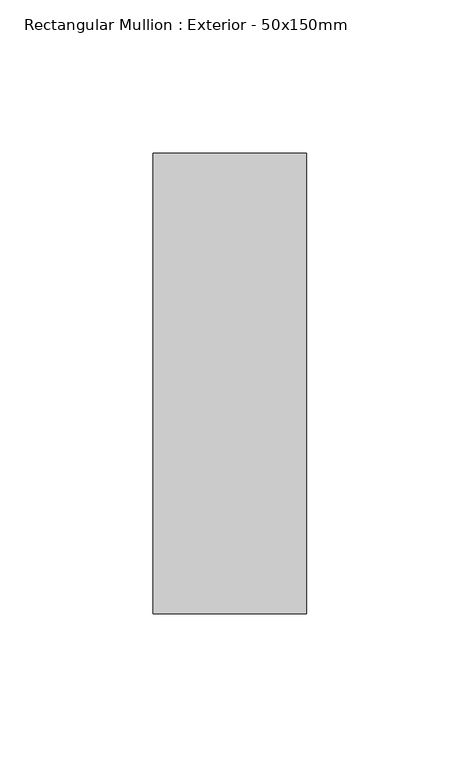
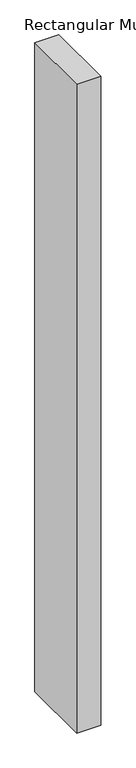
"""IFC4 building model written with IfcOpenShell, lengths in millimetres: member geometry, Rectangular Mullion : Exterior - 50x150mm."""

import ifcopenshell
import ifcopenshell.guid

model = None  # the IFC model being written
_history = None  # IfcOwnerHistory: only IFC2X3 demands one
_inside = {}  # id of a spatial element -> (the spatial element, [elements in it])
_under = {}  # id of a project, library or spatial element -> (it, [spatial elements below it])
_declared = {}  # id of a project -> (the project, [libraries it declares])
_typed = {}  # id of a type object -> (the type object, [elements of that type])
_made_of = {}  # id of a material, layer set ... -> (it, [elements and type objects made of it])


def new_model(schema):
    """Start an empty IFC model of exactly this schema.

    Asked for "IFC4X3", IfcOpenShell would pick the latest addendum, in which some entities
    have other attributes; the version numbers below select the first issue.
    IFC2X3 requires an IfcOwnerHistory on every rooted entity: one is made here for all.
    """
    global model, _history
    if schema == "IFC4X3":
        model = ifcopenshell.file(schema_version=(4, 3, 0, 0))
    else:
        model = ifcopenshell.file(schema=schema)
    _inside.clear()
    _under.clear()
    _declared.clear()
    _typed.clear()
    _made_of.clear()
    _history = None
    if model.schema == "IFC2X3":
        org = make("IfcOrganization", Name="unknown")
        user = make(
            "IfcPersonAndOrganization",
            ThePerson=make("IfcPerson", FamilyName="unknown"),
            TheOrganization=org,
        )
        app = make(
            "IfcApplication",
            ApplicationDeveloper=org,
            Version="unknown",
            ApplicationFullName="unknown",
            ApplicationIdentifier="unknown",
        )
        _history = make(
            "IfcOwnerHistory",
            OwningUser=user,
            OwningApplication=app,
            ChangeAction="ADDED",
            CreationDate=0,
        )
    return model


def make(cls, **values):
    """One entity of the class cls with the attributes given. An attribute that is None is left unset."""
    return model.create_entity(
        cls, **{name: value for name, value in values.items() if value is not None}
    )


def rooted(cls, **values):
    """An entity with a GlobalId (a new one), such as an element, a storey or a relation."""
    return make(cls, GlobalId=ifcopenshell.guid.new(), OwnerHistory=_history, **values)


def si_unit(unit_type, name, prefix=None):
    """IfcSIUnit, for example si_unit("LENGTHUNIT", "METRE", prefix="MILLI")."""
    return make("IfcSIUnit", UnitType=unit_type, Prefix=prefix, Name=name)


def assignment(units):
    """IfcUnitAssignment: the units of a project."""
    return None if units is None else make("IfcUnitAssignment", Units=units)


def point(xyz):
    """IfcCartesianPoint."""
    return None if xyz is None else make("IfcCartesianPoint", Coordinates=xyz)


def direction(xyz):
    """IfcDirection."""
    return None if xyz is None else make("IfcDirection", DirectionRatios=xyz)


def frame(location, z_axis=None, x_axis=None):
    """IfcAxis2Placement3D, a coordinate frame: its origin and axes. An axis left out is left unset."""
    return make(
        "IfcAxis2Placement3D",
        Location=point(location),
        Axis=direction(z_axis),
        RefDirection=direction(x_axis),
    )


def origin():
    """The frame at (0, 0, 0) with its axes left unset."""
    return frame((0.0, 0.0, 0.0))


def place(relative_to, where):
    """IfcLocalPlacement: puts the frame where relative to a parent placement (None: the world)."""
    return make(
        "IfcLocalPlacement", PlacementRelTo=relative_to, RelativePlacement=where
    )


def context(
    kind, dimensions, precision=None, world=None, true_north=None, identifier=None
):
    """IfcGeometricRepresentationContext, for example the 3D "Model" context."""
    return make(
        "IfcGeometricRepresentationContext",
        ContextIdentifier=identifier,
        ContextType=kind,
        CoordinateSpaceDimension=dimensions,
        Precision=precision,
        WorldCoordinateSystem=world,
        TrueNorth=true_north,
    )


def project(units=None, contexts=None):
    """IfcProject with its units and contexts."""
    return rooted(
        "IfcProject",
        Name="project",
        RepresentationContexts=contexts,
        UnitsInContext=assignment(units),
    )


def spatial(cls, under=None, at=None, **own):
    """A site, building, storey or space (cls), placed at a placement, below another one or the project."""
    s = rooted(cls, ObjectPlacement=at, **own)
    if under is not None:
        _under.setdefault(under.id(), (under, []))[1].append(s)
    return s


def polyline(points):
    """IfcPolyline through the points."""
    return make("IfcPolyline", Points=[point(p) for p in points])


def outline(outer, holes=None, kind="AREA"):
    """IfcArbitraryClosedProfileDef: a profile drawn as a closed curve; with holes, ...WithVoids."""
    if holes is None:
        return make("IfcArbitraryClosedProfileDef", ProfileType=kind, OuterCurve=outer)
    return make(
        "IfcArbitraryProfileDefWithVoids",
        ProfileType=kind,
        OuterCurve=outer,
        InnerCurves=holes,
    )


def extrude(swept, where, along, depth):
    """IfcExtrudedAreaSolid: the profile swept, set in the frame where, extruded along a direction by depth."""
    return make(
        "IfcExtrudedAreaSolid",
        SweptArea=swept,
        Position=where,
        ExtrudedDirection=direction(along),
        Depth=depth,
    )


def shape(context_of_items, identifier, shape_type, items):
    """IfcShapeRepresentation: the items that make up one representation, for example the "Body"."""
    return make(
        "IfcShapeRepresentation",
        ContextOfItems=context_of_items,
        RepresentationIdentifier=identifier,
        RepresentationType=shape_type,
        Items=items,
    )


def source(mapping_origin, context_of_items, identifier, shape_type, items):
    """IfcRepresentationMap: a shape defined once, which mapped items show again and again."""
    return make(
        "IfcRepresentationMap",
        MappingOrigin=mapping_origin,
        MappedRepresentation=shape(context_of_items, identifier, shape_type, items),
    )


def transform(
    local_origin,
    x_axis=None,
    y_axis=None,
    z_axis=None,
    scale=None,
    scale2=None,
    scale3=None,
    uniform=True,
):
    """IfcCartesianTransformationOperator3D, or its non-uniform kind. x_axis, y_axis, z_axis: its Axis1, 2, 3."""
    if uniform:
        return make(
            "IfcCartesianTransformationOperator3D",
            Axis1=direction(x_axis),
            Axis2=direction(y_axis),
            LocalOrigin=point(local_origin),
            Scale=scale,
            Axis3=direction(z_axis),
        )
    return make(
        "IfcCartesianTransformationOperator3DnonUniform",
        Axis1=direction(x_axis),
        Axis2=direction(y_axis),
        LocalOrigin=point(local_origin),
        Scale=scale,
        Axis3=direction(z_axis),
        Scale2=scale2,
        Scale3=scale3,
    )


def mapped(mapping_source, mapping_target):
    """IfcMappedItem: shows the shape of a source again, moved by a transform."""
    return make(
        "IfcMappedItem", MappingSource=mapping_source, MappingTarget=mapping_target
    )


def made_of(thing, what):
    """Note that an element or type object is made of a material, layer set ...; save() writes the relation."""
    if what is not None:
        _made_of.setdefault(what.id(), (what, []))[1].append(thing)
    return thing


def element(
    cls,
    number,
    at=None,
    inside=None,
    cuts=None,
    type_object=None,
    material=None,
    context=None,
    identifier="Body",
    shape_type=None,
    held_by="IfcProductDefinitionShape",
    body=None,
    shapes=None,
    **own,
):
    """One element of the class cls, such as IfcWall. Its Tag is "e" and its number.

    at: its placement. inside: the storey or other place that contains it. cuts: it is an
    opening in that element (IfcRelVoidsElement). A single representation is given by context,
    identifier, shape_type and body (its items); several are given by shapes. held_by: the class
    of the entity that holds the representations. save() writes the other relations.
    """
    e = rooted(cls, Tag="e%d" % number, ObjectPlacement=at, **own)
    if body is not None:
        shapes = [shape(context, identifier, shape_type, body)]
    if shapes is not None:
        e.Representation = make(held_by, Representations=shapes)
    if inside is not None:
        _inside.setdefault(inside.id(), (inside, []))[1].append(e)
    if cuts is not None:
        rooted(
            "IfcRelVoidsElement", RelatingBuildingElement=cuts, RelatedOpeningElement=e
        )
    if type_object is not None:
        _typed.setdefault(type_object.id(), (type_object, []))[1].append(e)
    return made_of(e, material)


def aggregate(whole, parts):
    """IfcRelAggregates: a whole, such as a stair, and the parts it consists of."""
    return rooted("IfcRelAggregates", RelatingObject=whole, RelatedObjects=parts)


def save(model, path):
    """Write the relations noted so far, then the file.

    IfcRelAggregates (storeys below a building ...), IfcRelContainedInSpatialStructure (elements
    in a storey), IfcRelDefinesByType, IfcRelAssociatesMaterial and IfcRelDeclares: one each for
    every whole, place, type object, material and project.
    """
    for whole, parts in _under.values():
        aggregate(whole, parts)
    for where, things in _inside.values():
        rooted(
            "IfcRelContainedInSpatialStructure",
            RelatedElements=things,
            RelatingStructure=where,
        )
    for kind, things in _typed.values():
        rooted("IfcRelDefinesByType", RelatedObjects=things, RelatingType=kind)
    for what, things in _made_of.values():
        rooted("IfcRelAssociatesMaterial", RelatedObjects=things, RelatingMaterial=what)
    for by, libraries in _declared.values():
        rooted("IfcRelDeclares", RelatingContext=by, RelatedDefinitions=libraries)
    model.write(path)


def rectangular_mullion_exterior_50x150mm_b89aef2e(model_context):
    return source(origin(), model_context, "Body", "SweptSolid", [
        extrude(outline(polyline([(0.0, 0.0), (0.0, -150.0), (-50.0, -150.0), (-50.0, 0.0), (0.0, 0.0)])), frame((0.0, 0.0, -1425.0000002), z_axis=(0.0, 0.0, 1.0), x_axis=(1.0, 0.0, 0.0)), (0.0, 0.0, 1.0), 1425.0000002),
    ])


if __name__ == "__main__":
    model = new_model("IFC4")
    model_context = context("Model", 3, world=origin())
    ifc_project = project(units=[si_unit("LENGTHUNIT", "METRE", prefix="MILLI")], contexts=[model_context])
    site = spatial("IfcSite", under=ifc_project)
    building = spatial("IfcBuilding", under=site)
    placement = place(None, origin())
    rectangular_mullion_exterior_50x150mm_shape = rectangular_mullion_exterior_50x150mm_b89aef2e(model_context)
    element("IfcMember", 1, ObjectType="Rectangular Mullion : Exterior - 50x150mm", at=placement, inside=building, context=model_context, shape_type="MappedRepresentation", body=[
        mapped(rectangular_mullion_exterior_50x150mm_shape, transform((0.0, 0.0, 0.0), x_axis=(1.0, 0.0, 0.0), y_axis=(0.0, 1.0, 0.0), z_axis=(0.0, 0.0, 1.0))),
    ])
    save(model, "model.ifc")

# Revit data of these elements
# Project information
#   Template Version = "DanEDU Building template ver. 2018.0420.0"
#   Client Name = "Test Project"
#   Project Address = "Enter address here"
#   Project Name = "3 Stories"
#   Project Number = "Number"
#   Current Version = "0.0.0"
#   SR Document GUID = "3eb9317e-835d-4f79-8926-4d15b96bc824"
# Type "Rectangular Mullion : Exterior - 50x150mm"
#   built-in parameter 1007351 = -0.246063 (stored number, unit not read)
#   built-in parameter 1007304 = 0.492126 (stored number, unit not read)
#   built-in parameter 1007301 = 0.082021 (stored number, unit not read)
#   built-in parameter 1007300 = 0.082021 (stored number, unit not read)
# Element 1 (IfcMember, "Rectangular Mullion : Exterior - 50x150mm")
#   Materials on its faces: "Default Frame/Mullion (Interior/Exterior)"
# Materials
#   "Default Frame/Mullion (Interior/Exterior)": class "Generic", colour RGB 205 205 205, transparency 0, Description = "Udefineret karm/ramme materiale", Cost = 0
